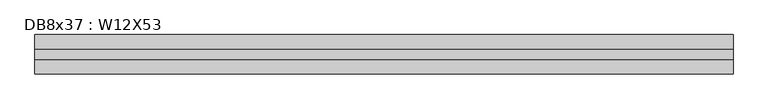
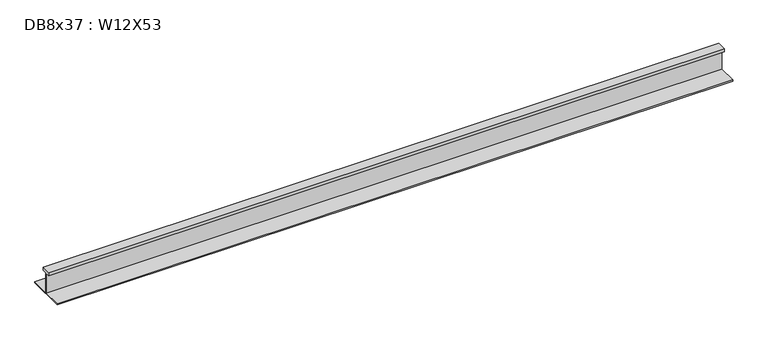
"""IFC4 building model written with IfcOpenShell, lengths in millimetres: beam geometry, DB8x37 : W12X53."""

from ifc_helpers import new_model, si_unit, frame, origin, place, context, project, spatial, polyline, outline, extrude, source, transform, mapped, element, save


def db8x37_w12x53_c743f8de(model_context):
    return source(origin(), model_context, "Body", "SweptSolid", [
        extrude(outline(polyline([(38.1, 145.415), (38.1, 120.015), (2.921, 120.015), (2.921, -48.4505), (152.4, -48.4505), (152.4, -58.1025), (-152.4, -58.1025), (-152.4, -48.4505), (-2.921, -48.4505), (-2.921, 120.015), (-38.1, 120.015), (-38.1, 145.415), (38.1, 145.415)])), frame((-2743.2, 0.0, 0.0), z_axis=(1.0, 0.0, 0.0), x_axis=(0.0, 1.0, 0.0)), (0.0, 0.0, 1.0), 5383.53),
    ])


if __name__ == "__main__":
    model = new_model("IFC4")
    model_context = context("Model", 3, world=origin())
    ifc_project = project(units=[si_unit("LENGTHUNIT", "METRE", prefix="MILLI")], contexts=[model_context])
    site = spatial("IfcSite", under=ifc_project)
    building = spatial("IfcBuilding", under=site)
    placement = place(None, origin())
    db8x37_w12x53_shape = db8x37_w12x53_c743f8de(model_context)
    element("IfcBeam", 1, ObjectType="DB8x37 : W12X53", at=placement, inside=building, context=model_context, shape_type="MappedRepresentation", body=[
        mapped(db8x37_w12x53_shape, transform((0.0, 0.0, 0.0), x_axis=(1.0, 0.0, 0.0), y_axis=(0.0, 1.0, 0.0), z_axis=(0.0, 0.0, 1.0))),
    ])
    save(model, "model.ifc")

# Revit data of these elements
# Type "DB8x37 : W12X53"
#   Assembly Code = "B10"
#   W = 53
#   Length [instance default] = 5' - 0"
#   bf = 0' - 10"
#   d = 1' - 0.1"
#   k = 0' - 1 3/8"
#   k2 = 0' - 0.8"
#   tf = 0' - 0.575"
#   tw = 0' - 0.345"
#   A = 0.108333 SF
#   Structural Material [instance default] = Steel ASTM A992
# Element 1 (IfcBeam, "DB8x37 : W12X53")
#   Materials on its faces: "Steel ASTM A992"
# Materials
#   "Steel ASTM A992": class "Metal", colour RGB 199 199 199, transparency 0, Description = "Structural steel 50ksi", Cost = 0
